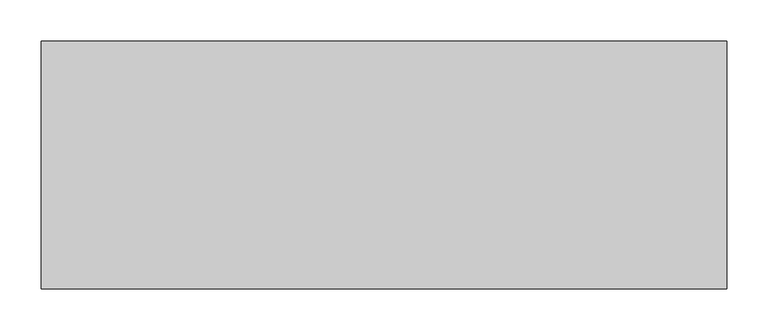
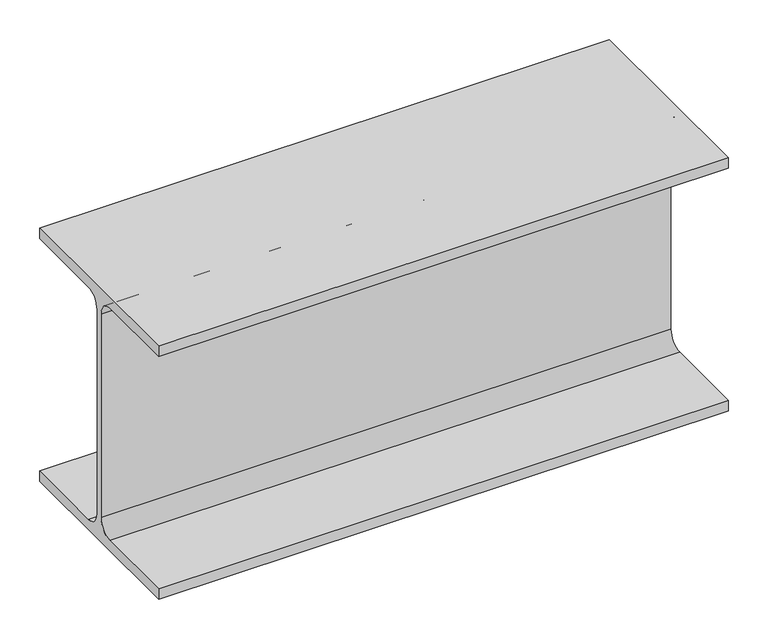
"""IFC4 building model written with IfcOpenShell, lengths in millimetres: beam geometry, 0912_Steel Framing_H-KSD3502 : H_SB_ASB_H-390x300x10x16."""

import ifcopenshell
import ifcopenshell.guid

model = None  # the IFC model being written
_history = None  # IfcOwnerHistory: only IFC2X3 demands one
_inside = {}  # id of a spatial element -> (the spatial element, [elements in it])
_under = {}  # id of a project, library or spatial element -> (it, [spatial elements below it])
_declared = {}  # id of a project -> (the project, [libraries it declares])
_typed = {}  # id of a type object -> (the type object, [elements of that type])
_made_of = {}  # id of a material, layer set ... -> (it, [elements and type objects made of it])


def new_model(schema):
    """Start an empty IFC model of exactly this schema.

    Asked for "IFC4X3", IfcOpenShell would pick the latest addendum, in which some entities
    have other attributes; the version numbers below select the first issue.
    IFC2X3 requires an IfcOwnerHistory on every rooted entity: one is made here for all.
    """
    global model, _history
    if schema == "IFC4X3":
        model = ifcopenshell.file(schema_version=(4, 3, 0, 0))
    else:
        model = ifcopenshell.file(schema=schema)
    _inside.clear()
    _under.clear()
    _declared.clear()
    _typed.clear()
    _made_of.clear()
    _history = None
    if model.schema == "IFC2X3":
        org = make("IfcOrganization", Name="unknown")
        user = make(
            "IfcPersonAndOrganization",
            ThePerson=make("IfcPerson", FamilyName="unknown"),
            TheOrganization=org,
        )
        app = make(
            "IfcApplication",
            ApplicationDeveloper=org,
            Version="unknown",
            ApplicationFullName="unknown",
            ApplicationIdentifier="unknown",
        )
        _history = make(
            "IfcOwnerHistory",
            OwningUser=user,
            OwningApplication=app,
            ChangeAction="ADDED",
            CreationDate=0,
        )
    return model


def make(cls, **values):
    """One entity of the class cls with the attributes given. An attribute that is None is left unset."""
    return model.create_entity(
        cls, **{name: value for name, value in values.items() if value is not None}
    )


def rooted(cls, **values):
    """An entity with a GlobalId (a new one), such as an element, a storey or a relation."""
    return make(cls, GlobalId=ifcopenshell.guid.new(), OwnerHistory=_history, **values)


def si_unit(unit_type, name, prefix=None):
    """IfcSIUnit, for example si_unit("LENGTHUNIT", "METRE", prefix="MILLI")."""
    return make("IfcSIUnit", UnitType=unit_type, Prefix=prefix, Name=name)


def assignment(units):
    """IfcUnitAssignment: the units of a project."""
    return None if units is None else make("IfcUnitAssignment", Units=units)


def point(xyz):
    """IfcCartesianPoint."""
    return None if xyz is None else make("IfcCartesianPoint", Coordinates=xyz)


def direction(xyz):
    """IfcDirection."""
    return None if xyz is None else make("IfcDirection", DirectionRatios=xyz)


def frame(location, z_axis=None, x_axis=None):
    """IfcAxis2Placement3D, a coordinate frame: its origin and axes. An axis left out is left unset."""
    return make(
        "IfcAxis2Placement3D",
        Location=point(location),
        Axis=direction(z_axis),
        RefDirection=direction(x_axis),
    )


def frame_2d(location, x_axis=None):
    """IfcAxis2Placement2D, a coordinate frame in the plane: its origin and x axis."""
    return make(
        "IfcAxis2Placement2D", Location=point(location), RefDirection=direction(x_axis)
    )


def origin():
    """The frame at (0, 0, 0) with its axes left unset."""
    return frame((0.0, 0.0, 0.0))


def place(relative_to, where):
    """IfcLocalPlacement: puts the frame where relative to a parent placement (None: the world)."""
    return make(
        "IfcLocalPlacement", PlacementRelTo=relative_to, RelativePlacement=where
    )


def context(
    kind, dimensions, precision=None, world=None, true_north=None, identifier=None
):
    """IfcGeometricRepresentationContext, for example the 3D "Model" context."""
    return make(
        "IfcGeometricRepresentationContext",
        ContextIdentifier=identifier,
        ContextType=kind,
        CoordinateSpaceDimension=dimensions,
        Precision=precision,
        WorldCoordinateSystem=world,
        TrueNorth=true_north,
    )


def project(units=None, contexts=None):
    """IfcProject with its units and contexts."""
    return rooted(
        "IfcProject",
        Name="project",
        RepresentationContexts=contexts,
        UnitsInContext=assignment(units),
    )


def spatial(cls, under=None, at=None, **own):
    """A site, building, storey or space (cls), placed at a placement, below another one or the project."""
    s = rooted(cls, ObjectPlacement=at, **own)
    if under is not None:
        _under.setdefault(under.id(), (under, []))[1].append(s)
    return s


def polyline(points):
    """IfcPolyline through the points."""
    return make("IfcPolyline", Points=[point(p) for p in points])


def circle_curve(where, radius):
    """IfcCircle in the frame where."""
    return make("IfcCircle", Position=where, Radius=radius)


def trimmed(basis, trim1, trim2, sense, master):
    """IfcTrimmedCurve: the piece of a basis curve between two trims."""
    return make(
        "IfcTrimmedCurve",
        BasisCurve=basis,
        Trim1=trim1,
        Trim2=trim2,
        SenseAgreement=sense,
        MasterRepresentation=master,
    )


def segment(curve, same_sense, transition):
    """IfcCompositeCurveSegment."""
    return make(
        "IfcCompositeCurveSegment",
        Transition=transition,
        SameSense=same_sense,
        ParentCurve=curve,
    )


def composite_curve(segments, self_intersect=None):
    """IfcCompositeCurve: segments joined end to end."""
    return make("IfcCompositeCurve", Segments=segments, SelfIntersect=self_intersect)


def outline(outer, holes=None, kind="AREA"):
    """IfcArbitraryClosedProfileDef: a profile drawn as a closed curve; with holes, ...WithVoids."""
    if holes is None:
        return make("IfcArbitraryClosedProfileDef", ProfileType=kind, OuterCurve=outer)
    return make(
        "IfcArbitraryProfileDefWithVoids",
        ProfileType=kind,
        OuterCurve=outer,
        InnerCurves=holes,
    )


def extrude(swept, where, along, depth):
    """IfcExtrudedAreaSolid: the profile swept, set in the frame where, extruded along a direction by depth."""
    return make(
        "IfcExtrudedAreaSolid",
        SweptArea=swept,
        Position=where,
        ExtrudedDirection=direction(along),
        Depth=depth,
    )


def shape(context_of_items, identifier, shape_type, items):
    """IfcShapeRepresentation: the items that make up one representation, for example the "Body"."""
    return make(
        "IfcShapeRepresentation",
        ContextOfItems=context_of_items,
        RepresentationIdentifier=identifier,
        RepresentationType=shape_type,
        Items=items,
    )


def source(mapping_origin, context_of_items, identifier, shape_type, items):
    """IfcRepresentationMap: a shape defined once, which mapped items show again and again."""
    return make(
        "IfcRepresentationMap",
        MappingOrigin=mapping_origin,
        MappedRepresentation=shape(context_of_items, identifier, shape_type, items),
    )


def transform(
    local_origin,
    x_axis=None,
    y_axis=None,
    z_axis=None,
    scale=None,
    scale2=None,
    scale3=None,
    uniform=True,
):
    """IfcCartesianTransformationOperator3D, or its non-uniform kind. x_axis, y_axis, z_axis: its Axis1, 2, 3."""
    if uniform:
        return make(
            "IfcCartesianTransformationOperator3D",
            Axis1=direction(x_axis),
            Axis2=direction(y_axis),
            LocalOrigin=point(local_origin),
            Scale=scale,
            Axis3=direction(z_axis),
        )
    return make(
        "IfcCartesianTransformationOperator3DnonUniform",
        Axis1=direction(x_axis),
        Axis2=direction(y_axis),
        LocalOrigin=point(local_origin),
        Scale=scale,
        Axis3=direction(z_axis),
        Scale2=scale2,
        Scale3=scale3,
    )


def mapped(mapping_source, mapping_target):
    """IfcMappedItem: shows the shape of a source again, moved by a transform."""
    return make(
        "IfcMappedItem", MappingSource=mapping_source, MappingTarget=mapping_target
    )


def made_of(thing, what):
    """Note that an element or type object is made of a material, layer set ...; save() writes the relation."""
    if what is not None:
        _made_of.setdefault(what.id(), (what, []))[1].append(thing)
    return thing


def element(
    cls,
    number,
    at=None,
    inside=None,
    cuts=None,
    type_object=None,
    material=None,
    context=None,
    identifier="Body",
    shape_type=None,
    held_by="IfcProductDefinitionShape",
    body=None,
    shapes=None,
    **own,
):
    """One element of the class cls, such as IfcWall. Its Tag is "e" and its number.

    at: its placement. inside: the storey or other place that contains it. cuts: it is an
    opening in that element (IfcRelVoidsElement). A single representation is given by context,
    identifier, shape_type and body (its items); several are given by shapes. held_by: the class
    of the entity that holds the representations. save() writes the other relations.
    """
    e = rooted(cls, Tag="e%d" % number, ObjectPlacement=at, **own)
    if body is not None:
        shapes = [shape(context, identifier, shape_type, body)]
    if shapes is not None:
        e.Representation = make(held_by, Representations=shapes)
    if inside is not None:
        _inside.setdefault(inside.id(), (inside, []))[1].append(e)
    if cuts is not None:
        rooted(
            "IfcRelVoidsElement", RelatingBuildingElement=cuts, RelatedOpeningElement=e
        )
    if type_object is not None:
        _typed.setdefault(type_object.id(), (type_object, []))[1].append(e)
    return made_of(e, material)


def aggregate(whole, parts):
    """IfcRelAggregates: a whole, such as a stair, and the parts it consists of."""
    return rooted("IfcRelAggregates", RelatingObject=whole, RelatedObjects=parts)


def save(model, path):
    """Write the relations noted so far, then the file.

    IfcRelAggregates (storeys below a building ...), IfcRelContainedInSpatialStructure (elements
    in a storey), IfcRelDefinesByType, IfcRelAssociatesMaterial and IfcRelDeclares: one each for
    every whole, place, type object, material and project.
    """
    for whole, parts in _under.values():
        aggregate(whole, parts)
    for where, things in _inside.values():
        rooted(
            "IfcRelContainedInSpatialStructure",
            RelatedElements=things,
            RelatingStructure=where,
        )
    for kind, things in _typed.values():
        rooted("IfcRelDefinesByType", RelatedObjects=things, RelatingType=kind)
    for what, things in _made_of.values():
        rooted("IfcRelAssociatesMaterial", RelatedObjects=things, RelatingMaterial=what)
    for by, libraries in _declared.values():
        rooted("IfcRelDeclares", RelatingContext=by, RelatedDefinitions=libraries)
    model.write(path)


def beam_b61b1237(model_context):
    return source(origin(), model_context, "Body", "SweptSolid", [
        extrude(outline(composite_curve([segment(polyline([(150.0, -179.0), (150.0, -195.0), (-150.0, -195.0), (-150.0, -179.0), (-27.0, -179.0)]), True, "CONTINUOUS"), segment(trimmed(circle_curve(frame_2d((-27.0, -157.0)), 22.0), [point((-27.0, -179.0))], [point((-5.0, -157.0))], True, "CARTESIAN"), True, "CONTINUOUS"), segment(polyline([(-5.0, -157.0), (-5.0, 157.0)]), True, "CONTINUOUS"), segment(trimmed(circle_curve(frame_2d((-27.0, 157.0)), 22.0), [point((-5.0, 157.0))], [point((-27.0, 179.0))], True, "CARTESIAN"), True, "CONTINUOUS"), segment(polyline([(-27.0, 179.0), (-150.0, 179.0), (-150.0, 195.0), (150.0, 195.0), (150.0, 179.0), (27.0, 179.0)]), True, "CONTINUOUS"), segment(trimmed(circle_curve(frame_2d((27.0, 157.0)), 22.0), [point((27.0, 179.0))], [point((5.0, 157.0))], True, "CARTESIAN"), True, "CONTINUOUS"), segment(polyline([(5.0, 157.0), (5.0, -157.0)]), True, "CONTINUOUS"), segment(trimmed(circle_curve(frame_2d((27.0, -157.0)), 22.0), [point((5.0, -157.0))], [point((27.0, -179.0))], True, "CARTESIAN"), True, "CONTINUOUS"), segment(polyline([(27.0, -179.0), (150.0, -179.0)]), True, "CONTINUOUS")], self_intersect=False)), frame((-415.0, 0.0, 0.0), z_axis=(1.0, 0.0, 0.0), x_axis=(0.0, 1.0, 0.0)), (0.0, 0.0, 1.0), 830.0),
    ])


if __name__ == "__main__":
    model = new_model("IFC4")
    model_context = context("Model", 3, world=origin())
    ifc_project = project(units=[si_unit("LENGTHUNIT", "METRE", prefix="MILLI")], contexts=[model_context])
    site = spatial("IfcSite", under=ifc_project)
    building = spatial("IfcBuilding", under=site)
    placement = place(None, origin())
    beam_shape = beam_b61b1237(model_context)
    element("IfcBeam", 1, ObjectType="0912_Steel Framing_H-KSD3502 : H_SB_ASB_H-390x300x10x16", at=placement, inside=building, context=model_context, shape_type="MappedRepresentation", body=[
        mapped(beam_shape, transform((0.0, 0.0, 0.0), x_axis=(1.0, 0.0, 0.0), y_axis=(0.0, 1.0, 0.0), z_axis=(0.0, 0.0, 1.0))),
    ])
    save(model, "model.ifc")

# Revit data of these elements
# Type "0912_Steel Framing_H-KSD3502 : H_SB_ASB_H-390x300x10x16"
#   H_WM Code_1 = "S01AA001-00001 | Main Steel Structure Fabrication Work | Shelter/Building | Heavy Steel - Standard (Weight≥90KG/M) | Material: (   )"
#   H_WM Code_2 = "S03AA027-00001 | Main Steel Structure Erection Work | Shelter/Building | Heavy Steel (Weight≥90KG/M) | Material: (   )"
#   H_WM Code_3 = "S01AA010-00001 | Main Steel Structure Fabrication Work | Shelter/Building | Steel Painting/Coating | for Non-Fireproofed Steel Surface, Surface Preparation, Primer, Second & Final Coat | Material: (   )"
#   H_Q'ty Cal Type Tag = "SB-Q2"
#   Width = 30.0 cm
#   Web Thickness = 1.0 cm
#   Web Fillet = 2.2 cm
#   Warping Constant = 2520000.0 cm⁶
#   W = 0
#   Torsional Moment of Inertia = 94.3867 cm⁴
#   Section Area = 136.0 cm²
#   Plastic Modulus weak axis = 733.0 cm³
#   Plastic Modulus strong axis = 2190.0 cm³
#   Perimeter = 1.92 m²/m
#   Nominal Weight = 107.00 kgf/m
#   Moment of Inertia weak axis = 7210.00 cm⁴
#   Moment of Inertia strong axis = 38700.00 cm⁴
#   Height = 39.0 cm
#   Flange Thickness = 1.6 cm
#   Elastic Modulus weak axis = 481.0 cm³
#   Elastic Modulus strong axis = 1980.0 cm³
#   Centroid Vertical = 19.5 cm
#   Centroid Horizontal = 15.0 cm
#   Ix = 387000000
#   Length [instance default] = 1.5240 m
#   Zx = 2190000
#   b = 0.3000 m
#   h = 0.3900 m
#   r = 0.0220 m
#   s = 0.0100 m
#   t = 0.0160 m
#   A = 0.0136 m²
#   Structural Material [instance default] = Steel, 45-345
#   Assembly Code = ""
# Element 1 (IfcBeam, "0912_Steel Framing_H-KSD3502 : H_SB_ASB_H-390x300x10x16")
#   Structural Material = none
# Materials
#   "Steel, 45-345": class "Metal", colour RGB 189 187 185, transparency 0, Description = "Steel 345 MPa", Cost = 0
